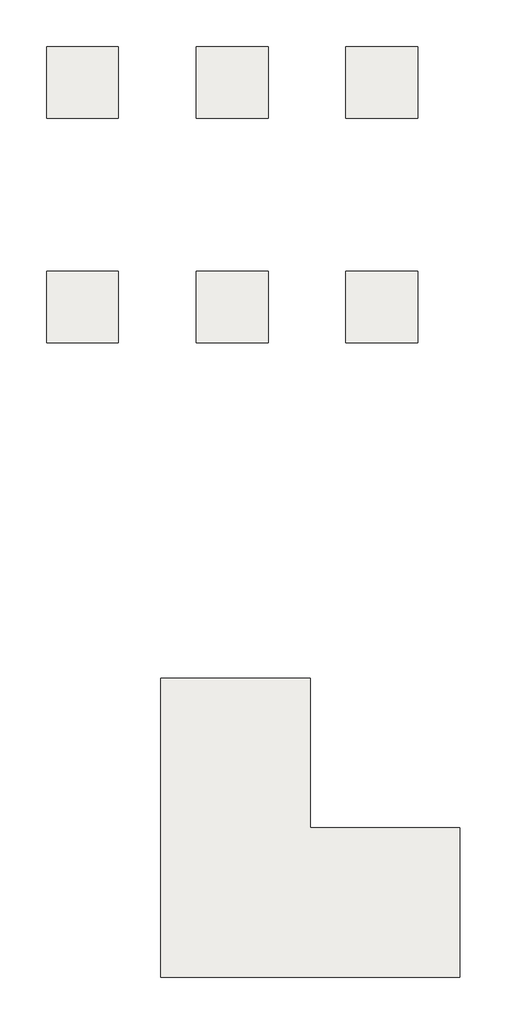
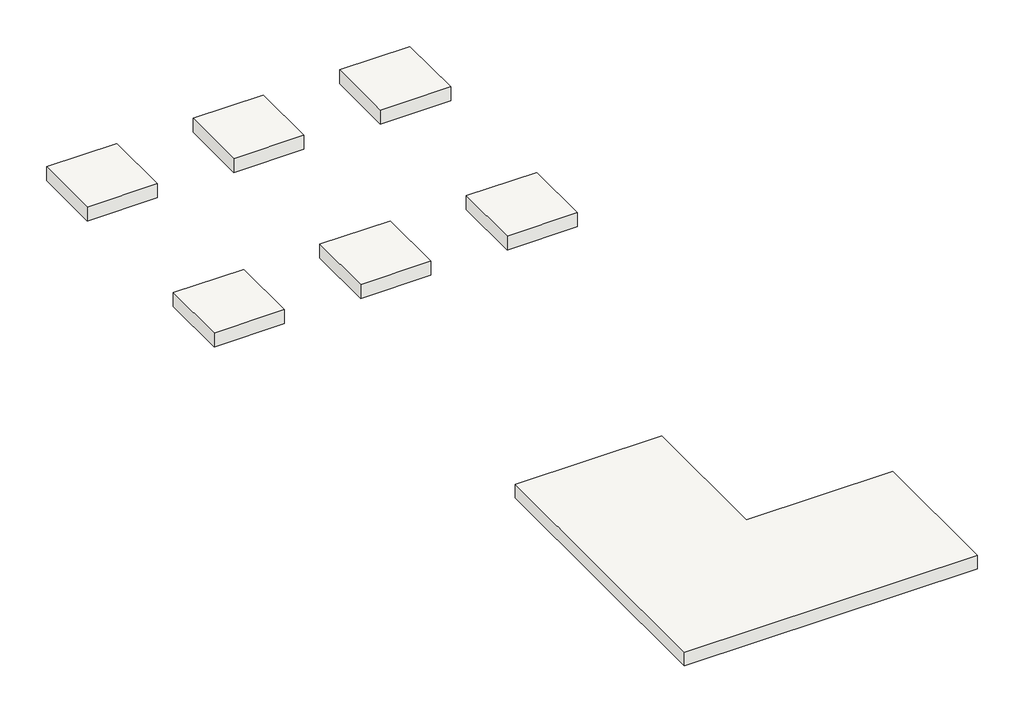
# Not in any storey: 7 slabs.
"""IFC4 building model written with IfcOpenShell, lengths in millimetres."""

from ifc_helpers import new_model, si_unit, frame, origin, place, context, project, spatial, polyline, outline, extrude, element, save

model = new_model("IFC4")

# Units and contexts
model_context = context("Model", 3, world=origin())
ifc_project = project(units=[si_unit("LENGTHUNIT", "METRE", prefix="MILLI")], contexts=[model_context])

# Site, building
site = spatial("IfcSite", under=ifc_project)
building = spatial("IfcBuilding", under=site)

# Slabs
placement = place(None, origin())
element("IfcSlab", 1, ObjectType="FT211-Footing-Rectangular_void test : FT211_10000x10000x500_test", at=placement, inside=building, context=model_context, shape_type="SweptSolid", body=[
    extrude(outline(polyline([(12612.0, -8900.4608631), (2612.0, -8900.4608631), (2612.0, 1099.5391369), (7612.0, 1099.5391369), (7612.0, -3900.4608631), (12612.0, -3900.4608631), (12612.0, -8900.4608631)])), frame((0.0, 0.0, -1800.0), z_axis=(0.0, 0.0, 1.0), x_axis=(1.0, 0.0, 0.0)), (0.0, 0.0, 1.0), 500.0),
])
element("IfcSlab", 2, ObjectType="FT211-Footing-Rectangular_더미삭제 : FT211_2400x2400x500", at=placement, inside=building, context=model_context, shape_type="SweptSolid", body=[
    extrude(outline(polyline([(6200.0, 14699.5208589), (6200.0, 12299.5208589), (3800.0, 12299.5208589), (3800.0, 14699.5208589), (6200.0, 14699.5208589)])), frame((0.0, 0.0, -1800.0), z_axis=(0.0, 0.0, 1.0), x_axis=(1.0, 0.0, 0.0)), (0.0, 0.0, 1.0), 500.0),
])
element("IfcSlab", 3, ObjectType="FT211-Footing-Rectangular_더미삭제 : FT211_2400x2400x500", at=placement, inside=building, context=model_context, shape_type="SweptSolid", body=[
    extrude(outline(polyline([(11200.0, 14699.5208589), (11200.0, 12299.5208589), (8800.0, 12299.5208589), (8800.0, 14699.5208589), (11200.0, 14699.5208589)])), frame((0.0, 0.0, -1800.0), z_axis=(0.0, 0.0, 1.0), x_axis=(1.0, 0.0, 0.0)), (0.0, 0.0, 1.0), 500.0),
])
element("IfcSlab", 4, ObjectType="FT211-Footing-Rectangular_더미삭제 : FT211_2400x2400x500", at=placement, inside=building, context=model_context, shape_type="SweptSolid", body=[
    extrude(outline(polyline([(11200.0, 22199.5208589), (11200.0, 19799.5208589), (8800.0, 19799.5208589), (8800.0, 22199.5208589), (11200.0, 22199.5208589)])), frame((0.0, 0.0, -1800.0), z_axis=(0.0, 0.0, 1.0), x_axis=(1.0, 0.0, 0.0)), (0.0, 0.0, 1.0), 500.0),
])
element("IfcSlab", 5, ObjectType="FT211-Footing-Rectangular_더미삭제 : FT211_2400x2400x500", at=placement, inside=building, context=model_context, shape_type="SweptSolid", body=[
    extrude(outline(polyline([(6200.0, 22199.5208589), (6200.0, 19799.5208589), (3800.0, 19799.5208589), (3800.0, 22199.5208589), (6200.0, 22199.5208589)])), frame((0.0, 0.0, -1800.0), z_axis=(0.0, 0.0, 1.0), x_axis=(1.0, 0.0, 0.0)), (0.0, 0.0, 1.0), 500.0),
])
element("IfcSlab", 6, ObjectType="FT211-Footing-Rectangular_더미삭제 : FT211_2400x2400x500", at=placement, inside=building, context=model_context, shape_type="SweptSolid", body=[
    extrude(outline(polyline([(1200.0, 22199.5208589), (1200.0, 19799.5208589), (-1200.0, 19799.5208589), (-1200.0, 22199.5208589), (1200.0, 22199.5208589)])), frame((0.0, 0.0, -1800.0), z_axis=(0.0, 0.0, 1.0), x_axis=(1.0, 0.0, 0.0)), (0.0, 0.0, 1.0), 500.0),
])
element("IfcSlab", 7, ObjectType="FT211-Footing-Rectangular_더미삭제 : FT211_2400x2400x500", at=placement, inside=building, context=model_context, shape_type="SweptSolid", body=[
    extrude(outline(polyline([(1200.0, 14699.5208589), (1200.0, 12299.5208589), (-1200.0, 12299.5208589), (-1200.0, 14699.5208589), (1200.0, 14699.5208589)])), frame((0.0, 0.0, -1800.0), z_axis=(0.0, 0.0, 1.0), x_axis=(1.0, 0.0, 0.0)), (0.0, 0.0, 1.0), 500.0),
])

save(model, "model.ifc")

# Revit data of these elements
# Project information
#   Building Name = "MAIN GATE SECURITY BUILDING"
#   Project Status = "Project Status"
#   Client Name = "현대엔지니어링"
#   Project Address = "서울시 종로구 율곡로 75(계동)"
#   Project Name = "Therma Visayas Energy Project"
#   Project Number = "-"
# Grids (mm)
#   "A": line (0, 24502.793) -> (0, 11308.625)
#   "B": line (5000, 24502.793) -> (5000, 11308.625)
#   "C": line (10000, 24502.793) -> (10000, 11308.625)
#   "1": line (-3860.098, 13499.521) -> (12441.468, 13499.521)
#   "2": line (-3860.098, 20999.521) -> (12441.468, 20999.521)
# Type "FT211-Footing-Rectangular_void test : FT211_10000x10000x500_test"
#   Top bar = "D25@300"
#   Description = "UG Shallow Foundation"
#   Bottom bar = "D20@300"
#   Width = 10000 mm
#   Length = 10000 mm
#   Foundation Thickness = 500 mm
#   Structural Material [instance default] = A03AC032-00007_Structural Concrete_Type1_25MPa-30Mpa
#   Assembly Code = ""
# Type "FT211-Footing-Rectangular_더미삭제 : FT211_2400x2400x500"
#   Top bar = "D25@300"
#   Description = "UG Shallow Foundation"
#   Bottom bar = "D20@300"
#   Width = 2400 mm
#   Length = 2400 mm
#   Foundation Thickness = 500 mm
#   Structural Material [instance default] = A03AC032-00007_Structural Concrete_Type1_25MPa-30Mpa
#   Assembly Code = ""
# Element 1 (IfcSlab, "FT211-Footing-Rectangular_void test : FT211_10000x10000x500_test")
#   Comments = ""
#   Structural Material = A03AC032-00007_Structural Concrete_Type1_25MPa-30Mpa
#   Phase Created = New Construction
#   Materials on its faces: "A03AC032-00007_Structural Concrete_Type1_25MPa-30Mpa"
# Elements 2, 3, 4, 5, 6, 7 (IfcSlab, "FT211-Footing-Rectangular_더미삭제 : FT211_2400x2400x500")
#   Comments = ""
#   Mark = "F1"
#   F01) Building Name = "Main Gate House"
#   F11) Project Building Tag_Type-1 = "Common"
#   F12) Project Building Tag_Type-2 = "Common"
#   F13) Project Facility Code = "Facility Code"
#   F21) Structural Type = "Concrete"
#   F31) Standard Building Code = "IBC"
#   F41) Discipline = "AR"
#   F51) Plan Start Date-Engineering = "2015-01-01"
#   F52) Plan Finish Date-Engineering = "2015-12-31"
#   F53) Duration = "365"
#   F54) Actual Start Date-Engineering = "2015-01-01"
#   F55) Actual Finish Date-Engineering = "2015-12-31"
#   F61) Plan Start Date-Construction = "2016-08-19"
#   F62) Plan Finish Date-Construction = "2017-01-31"
#   F64) Actual Start Date-Construction = "2016-08-19"
#   F63) Duration = "202"
#   F65) Actual Finish Date-Construction = "2017-01-31"
#   F91) Plant Type = "CFPP"
#   F92) KKS Structures, Building = "UYF"
#   P01) Project Name = "TVEP"
#   P02) Project Configuration = "CFB Boiler x 2(Foster Wheeler) + STG x 2(Alstom, 150MW)"
#   P03) Project Abbreviation = "TVEP"
#   P04) Project Code = "BEPH1402"
#   P05) Project Stage = "In operation"
#   P06) Project Location = "Sito Looc, Barangay Bato, Toledo City in Philippines"
#   P07) Project Owner = "Therma Visayas, Inc."
#   P08) Project O.E = "Flour"
#   P09) Project Schedule = "ITB Issueing Date : 2013.07.30\r\nSite Survey : 2013.08.19-20\r\nBid Closing Date : 2013.11.29\r\nPreferred Bidder Notice 접수 : 2014.04.27\r\nTarget award date : 2014 05\r\nLOA 접수 : 2014.05.21\r\nSigning Ceremony : 2014.05.30"
#   P10) Basic Wind Speed = "55.6 m/s"
#   P11) Seismic = "NSCP 2010, Zone 4 (PGA : 0.4g)"
#   P12) Soil = "Sc"
#   P13) Soil Capacity = "100kN/m2"
#   P14) Pile Capacity = "PHC(D400) : 1200kN"
#   W00) Work Master Code = "A03AC032-00007"
#   W01) Work Master_Lv1 = "Concrete Work"
#   W02) Work Master_Lv2 = "Substructure Work"
#   W03) Work Master_Spec.1 = "Cement Type-1"
#   W04) Work Master_Spec.2 = "25MPa < F'c (Cylinder Strength) ≤ 30MPa"
#   W11) Activity ID = "C02AGB010"
#   W12) Activity Name = "Main Gate Security Building - Building Foundation"
#   W13) Plan Start Date = "2016-08-19"
#   W14) Plan Finish Date = "2016-09-22"
#   W15) Duration = "26"
#   W16) Actual Start Date = "2016-08-19"
#   W17) Actual Finish Date = "2016-09-22"
#   R02) Unit Price = 0
#   Structural Material = A03AC032-00007_Structural Concrete_Type1_25MPa-30Mpa
#   Phase Created = New Construction
#   Materials on its faces: "A03AC032-00007_Structural Concrete_Type1_25MPa-30Mpa"
# Materials
#   "A03AC032-00007_Structural Concrete_Type1_25MPa-30Mpa": class "Concrete", colour RGB 176 176 176, transparency 0, Keynote = "09910.A1", Description = "Reinf. Conc.", W00) Work Master Code = "A03AC032-00007", W01) Work Master_Lv1 = "Concrete Work", W02) Work Master_Lv2 = "Substructure Work", W03) Work Master_Spec.1 = "Structural Concrete", W04) Work Master_Spec.2 = "Cement Type-1", W05) Work Master_Spec.3 = "25MPa < F'c (Cylinder Strength) ≤ 30MPa", Cost = 0
